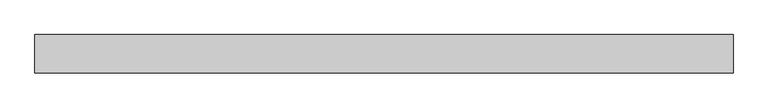
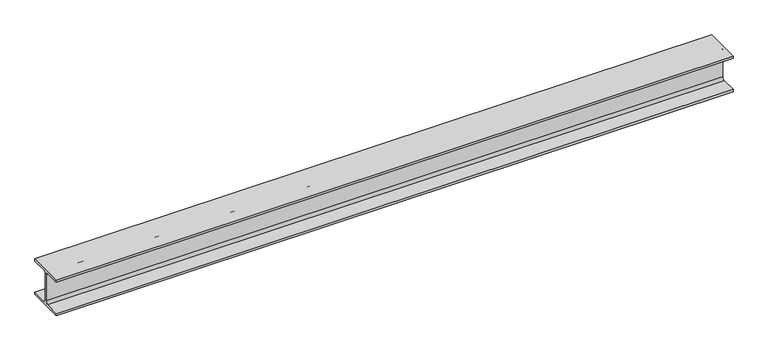
"""IFC4 building model written with IfcOpenShell, lengths in millimetres: beam geometry, 0912_Steel Framing_H-KSD3502 : H_SB_ASB_H-200x200x8x12."""

from ifc_helpers import new_model, si_unit, point, frame, frame_2d, origin, place, context, project, spatial, polyline, circle_curve, trimmed, segment, composite_curve, outline, extrude, source, transform, mapped, element, save


def beam_006f807e(model_context):
    return source(origin(), model_context, "Body", "SweptSolid", [
        extrude(outline(composite_curve([segment(polyline([(-100.0, -88.0), (-17.0, -88.0)]), True, "CONTINUOUS"), segment(trimmed(circle_curve(frame_2d((-17.0, -75.0)), 13.0), [point((-17.0, -88.0))], [point((-4.0, -75.0))], True, "CARTESIAN"), True, "CONTINUOUS"), segment(polyline([(-4.0, -75.0), (-4.0, 75.0)]), True, "CONTINUOUS"), segment(trimmed(circle_curve(frame_2d((-17.0, 75.0)), 13.0), [point((-4.0, 75.0))], [point((-17.0, 88.0))], True, "CARTESIAN"), True, "CONTINUOUS"), segment(polyline([(-17.0, 88.0), (-100.0, 88.0), (-100.0, 100.0), (100.0, 100.0), (100.0, 88.0), (17.0, 88.0)]), True, "CONTINUOUS"), segment(trimmed(circle_curve(frame_2d((17.0, 75.0)), 13.0), [point((17.0, 88.0))], [point((4.0, 75.0))], True, "CARTESIAN"), True, "CONTINUOUS"), segment(polyline([(4.0, 75.0), (4.0, -75.0)]), True, "CONTINUOUS"), segment(trimmed(circle_curve(frame_2d((17.0, -75.0)), 13.0), [point((4.0, -75.0))], [point((17.0, -88.0))], True, "CARTESIAN"), True, "CONTINUOUS"), segment(polyline([(17.0, -88.0), (100.0, -88.0), (100.0, -100.0), (-100.0, -100.0), (-100.0, -88.0)]), True, "CONTINUOUS")], self_intersect=False)), frame((-1827.2740995, 0.0, 0.0), z_axis=(1.0, 0.0, 0.0), x_axis=(0.0, 1.0, 0.0)), (0.0, 0.0, 1.0), 3629.4587666),
    ])


if __name__ == "__main__":
    model = new_model("IFC4")
    model_context = context("Model", 3, world=origin())
    ifc_project = project(units=[si_unit("LENGTHUNIT", "METRE", prefix="MILLI")], contexts=[model_context])
    site = spatial("IfcSite", under=ifc_project)
    building = spatial("IfcBuilding", under=site)
    placement = place(None, origin())
    beam_shape = beam_006f807e(model_context)
    element("IfcBeam", 1, ObjectType="0912_Steel Framing_H-KSD3502 : H_SB_ASB_H-200x200x8x12", at=placement, inside=building, context=model_context, shape_type="MappedRepresentation", body=[
        mapped(beam_shape, transform((0.0, 0.0, 0.0), x_axis=(1.0, 0.0, 0.0), y_axis=(0.0, 1.0, 0.0), z_axis=(0.0, 0.0, 1.0))),
    ])
    save(model, "model.ifc")

# Revit data of these elements
# Type "0912_Steel Framing_H-KSD3502 : H_SB_ASB_H-200x200x8x12"
#   H_WM Code_1 = "S01AA002-00001 | Main Steel Structure Fabrication Work | Shelter/Building | Medium Steel - Standard (90KG/M>Weight≥30KG/M) | Material: (   )"
#   H_WM Code_2 = "S03AA028-00001 | Main Steel Structure Erection Work | Shelter/Building | Medium Steel (90KG/M>Weight≥30KG/M) | Material: (   )"
#   H_WM Code_3 = "S01AA010-00001 | Main Steel Structure Fabrication Work | Shelter/Building | Steel Painting/Coating | for Non-Fireproofed Steel Surface, Surface Preparation, Primer, Second & Final Coat | Material: (   )"
#   H_Q'ty Cal Type Tag = "SB-Q2"
#   Width = 20.0 cm
#   Web Thickness = 0.8 cm
#   Web Fillet = 1.3 cm
#   Warping Constant = 141000.0 cm⁶
#   W = 0
#   Torsional Moment of Inertia = 26.2485 cm⁴
#   Section Area = 63.53 cm²
#   Plastic Modulus weak axis = 244.0 cm³
#   Plastic Modulus strong axis = 525.0 cm³
#   Perimeter = 1.16 m²/m
#   Nominal Weight = 49.90 kgf/m
#   Moment of Inertia weak axis = 1600.00 cm⁴
#   Moment of Inertia strong axis = 4720.00 cm⁴
#   Height = 20.0 cm
#   Flange Thickness = 1.2 cm
#   Elastic Modulus weak axis = 160.0 cm³
#   Elastic Modulus strong axis = 472.0 cm³
#   Centroid Vertical = 10.0 cm
#   Centroid Horizontal = 10.0 cm
#   Ix = 47200000
#   Length [instance default] = 1.5240 m
#   Zx = 525000
#   b = 0.2000 m
#   h = 0.2000 m
#   r = 0.0130 m
#   s = 0.0080 m
#   t = 0.0120 m
#   A = 0.006353 m²
#   Structural Material [instance default] = Steel, 45-345
#   Assembly Code = ""
# Element 1 (IfcBeam, "0912_Steel Framing_H-KSD3502 : H_SB_ASB_H-200x200x8x12")
#   Structural Material = none
# Materials
#   "Steel, 45-345": class "Metal", colour RGB 189 187 185, transparency 0, Description = "Steel 345 MPa", Cost = 0
